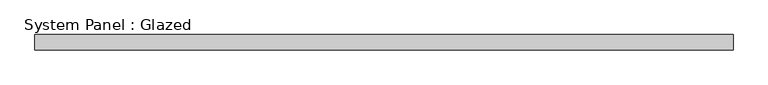
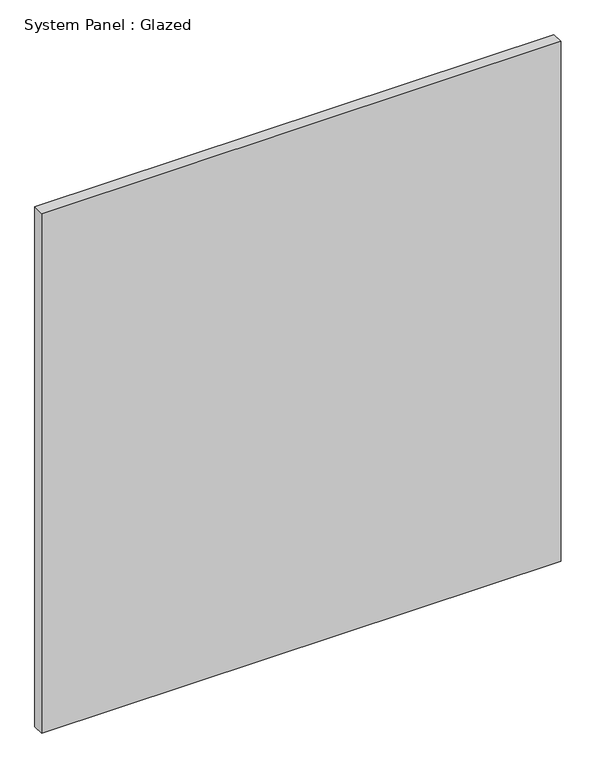
"""IFC4 building model written with IfcOpenShell, lengths in millimetres: plate geometry, System Panel : Glazed."""

from ifc_helpers import new_model, si_unit, origin, origin_with_axes, place, context, project, spatial, polyline, outline, extrude, source, transform, mapped, element, save


def system_panel_glazed_ab3c60aa(model_context):
    return source(origin(), model_context, "Body", "SweptSolid", [
        extrude(outline(polyline([(576.624914, 19.05), (-576.624914, 19.05), (-576.624914, 44.45), (576.624914, 44.45), (576.624914, 19.05)])), origin_with_axes(), (0.0, 0.0, 1.0), 1219.2),
    ])


if __name__ == "__main__":
    model = new_model("IFC4")
    model_context = context("Model", 3, world=origin())
    ifc_project = project(units=[si_unit("LENGTHUNIT", "METRE", prefix="MILLI")], contexts=[model_context])
    site = spatial("IfcSite", under=ifc_project)
    building = spatial("IfcBuilding", under=site)
    placement = place(None, origin())
    system_panel_glazed_shape = system_panel_glazed_ab3c60aa(model_context)
    element("IfcPlate", 1, ObjectType="System Panel : Glazed", at=placement, inside=building, context=model_context, shape_type="MappedRepresentation", body=[
        mapped(system_panel_glazed_shape, transform((0.0, 0.0, 0.0), x_axis=(1.0, 0.0, 0.0), y_axis=(0.0, 1.0, 0.0), z_axis=(0.0, 0.0, 1.0))),
    ])
    save(model, "model.ifc")

# Revit data of these elements
# Element 1 (IfcPlate, "System Panel : Glazed")
#   Materials on its faces: "Glass"
# Materials
#   "Glass": class "Glass", colour RGB 0 128 192, transparency 0.75
